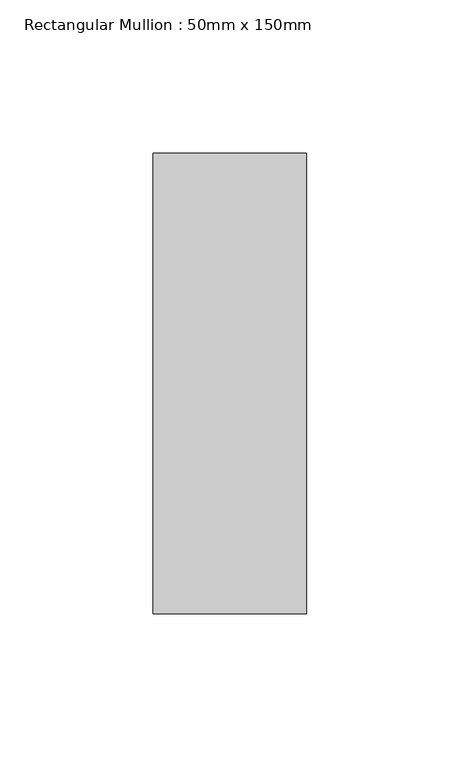
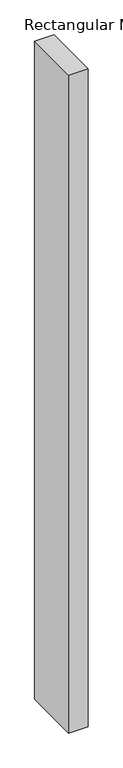
"""IFC4 building model written with IfcOpenShell, lengths in millimetres: member geometry, Rectangular Mullion : 50mm x 150mm."""

from ifc_helpers import new_model, si_unit, frame, origin, place, context, project, spatial, polyline, outline, extrude, source, transform, mapped, element, save


def rectangular_mullion_50mm_x_150mm_c1958830(model_context):
    return source(origin(), model_context, "Body", "SweptSolid", [
        extrude(outline(polyline([(0.0, 75.0), (0.0, -75.0), (-50.0, -75.0), (-50.0, 75.0), (0.0, 75.0)])), frame((0.0, 0.0, -1780.0000003), z_axis=(0.0, 0.0, 1.0), x_axis=(1.0, 0.0, 0.0)), (0.0, 0.0, 1.0), 1780.0000003),
    ])


if __name__ == "__main__":
    model = new_model("IFC4")
    model_context = context("Model", 3, world=origin())
    ifc_project = project(units=[si_unit("LENGTHUNIT", "METRE", prefix="MILLI")], contexts=[model_context])
    site = spatial("IfcSite", under=ifc_project)
    building = spatial("IfcBuilding", under=site)
    placement = place(None, origin())
    rectangular_mullion_50mm_x_150mm_shape = rectangular_mullion_50mm_x_150mm_c1958830(model_context)
    element("IfcMember", 1, ObjectType="Rectangular Mullion : 50mm x 150mm", at=placement, inside=building, context=model_context, shape_type="MappedRepresentation", body=[
        mapped(rectangular_mullion_50mm_x_150mm_shape, transform((0.0, 0.0, 0.0), x_axis=(1.0, 0.0, 0.0), y_axis=(0.0, 1.0, 0.0), z_axis=(0.0, 0.0, 1.0))),
    ])
    save(model, "model.ifc")

# Revit data of these elements
# Type "Rectangular Mullion : 50mm x 150mm"
#   built-in parameter 1007304 = 0.492126 (stored number, unit not read)
#   built-in parameter 1007301 = 0.082021 (stored number, unit not read)
#   built-in parameter 1007300 = 0.082021 (stored number, unit not read)
# Element 1 (IfcMember, "Rectangular Mullion : 50mm x 150mm")
#   Materials on its faces: "Aluminum"
# Materials
#   "Aluminum": class "Metal", colour RGB 244 244 244, transparency 0, Description = "Aluminum 6061", Cost = 0
